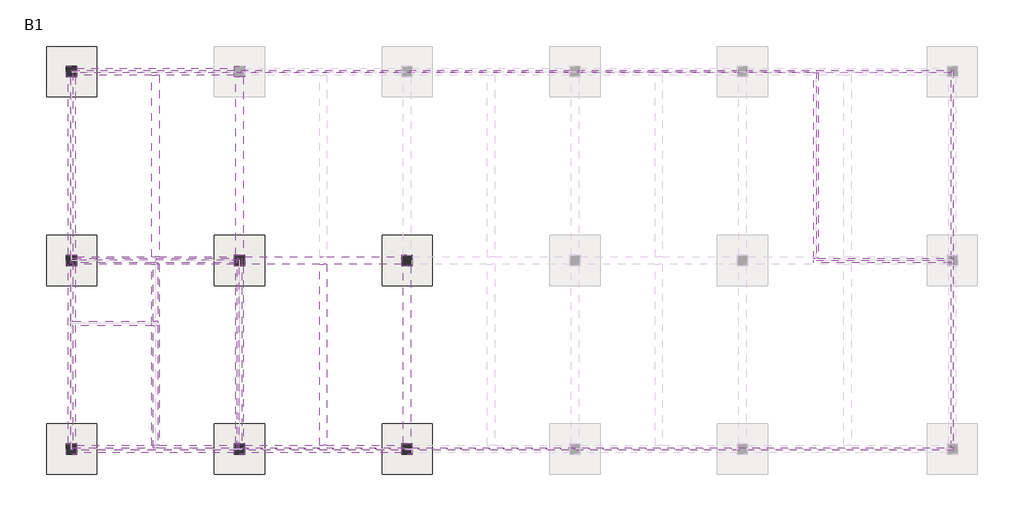
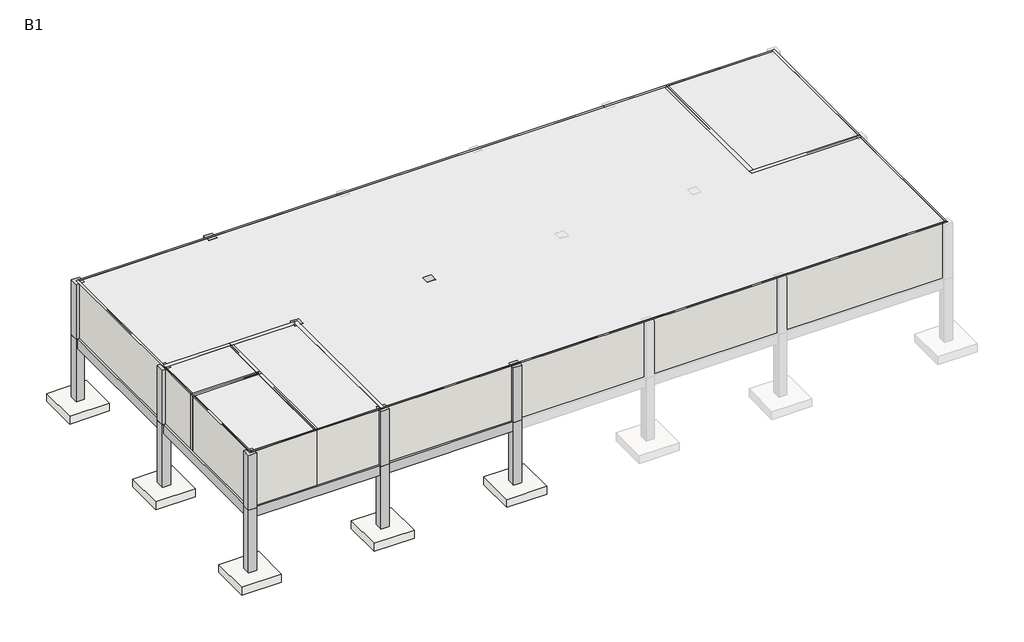
# One storey, part 1 of 2: 18 walls, 15 columns, 13 beams, 12 slabs.
"""IFC4 building model written with IfcOpenShell, lengths in millimetres."""

import ifcopenshell
import ifcopenshell.guid

model = None  # the IFC model being written
_history = None  # IfcOwnerHistory: only IFC2X3 demands one
_inside = {}  # id of a spatial element -> (the spatial element, [elements in it])
_under = {}  # id of a project, library or spatial element -> (it, [spatial elements below it])
_declared = {}  # id of a project -> (the project, [libraries it declares])
_typed = {}  # id of a type object -> (the type object, [elements of that type])
_made_of = {}  # id of a material, layer set ... -> (it, [elements and type objects made of it])


def new_model(schema):
    """Start an empty IFC model of exactly this schema.

    Asked for "IFC4X3", IfcOpenShell would pick the latest addendum, in which some entities
    have other attributes; the version numbers below select the first issue.
    IFC2X3 requires an IfcOwnerHistory on every rooted entity: one is made here for all.
    """
    global model, _history
    if schema == "IFC4X3":
        model = ifcopenshell.file(schema_version=(4, 3, 0, 0))
    else:
        model = ifcopenshell.file(schema=schema)
    _inside.clear()
    _under.clear()
    _declared.clear()
    _typed.clear()
    _made_of.clear()
    _history = None
    if model.schema == "IFC2X3":
        org = make("IfcOrganization", Name="unknown")
        user = make(
            "IfcPersonAndOrganization",
            ThePerson=make("IfcPerson", FamilyName="unknown"),
            TheOrganization=org,
        )
        app = make(
            "IfcApplication",
            ApplicationDeveloper=org,
            Version="unknown",
            ApplicationFullName="unknown",
            ApplicationIdentifier="unknown",
        )
        _history = make(
            "IfcOwnerHistory",
            OwningUser=user,
            OwningApplication=app,
            ChangeAction="ADDED",
            CreationDate=0,
        )
    return model


def make(cls, **values):
    """One entity of the class cls with the attributes given. An attribute that is None is left unset."""
    return model.create_entity(
        cls, **{name: value for name, value in values.items() if value is not None}
    )


def rooted(cls, **values):
    """An entity with a GlobalId (a new one), such as an element, a storey or a relation."""
    return make(cls, GlobalId=ifcopenshell.guid.new(), OwnerHistory=_history, **values)


def si_unit(unit_type, name, prefix=None):
    """IfcSIUnit, for example si_unit("LENGTHUNIT", "METRE", prefix="MILLI")."""
    return make("IfcSIUnit", UnitType=unit_type, Prefix=prefix, Name=name)


def assignment(units):
    """IfcUnitAssignment: the units of a project."""
    return None if units is None else make("IfcUnitAssignment", Units=units)


def point(xyz):
    """IfcCartesianPoint."""
    return None if xyz is None else make("IfcCartesianPoint", Coordinates=xyz)


def direction(xyz):
    """IfcDirection."""
    return None if xyz is None else make("IfcDirection", DirectionRatios=xyz)


def frame(location, z_axis=None, x_axis=None):
    """IfcAxis2Placement3D, a coordinate frame: its origin and axes. An axis left out is left unset."""
    return make(
        "IfcAxis2Placement3D",
        Location=point(location),
        Axis=direction(z_axis),
        RefDirection=direction(x_axis),
    )


def origin():
    """The frame at (0, 0, 0) with its axes left unset."""
    return frame((0.0, 0.0, 0.0))


def origin_with_axes():
    """The frame at (0, 0, 0) with the z axis (0, 0, 1) and the x axis (1, 0, 0) written out."""
    return frame((0.0, 0.0, 0.0), z_axis=(0.0, 0.0, 1.0), x_axis=(1.0, 0.0, 0.0))


def place(relative_to, where):
    """IfcLocalPlacement: puts the frame where relative to a parent placement (None: the world)."""
    return make(
        "IfcLocalPlacement", PlacementRelTo=relative_to, RelativePlacement=where
    )


def context(
    kind, dimensions, precision=None, world=None, true_north=None, identifier=None
):
    """IfcGeometricRepresentationContext, for example the 3D "Model" context."""
    return make(
        "IfcGeometricRepresentationContext",
        ContextIdentifier=identifier,
        ContextType=kind,
        CoordinateSpaceDimension=dimensions,
        Precision=precision,
        WorldCoordinateSystem=world,
        TrueNorth=true_north,
    )


def project(units=None, contexts=None):
    """IfcProject with its units and contexts."""
    return rooted(
        "IfcProject",
        Name="project",
        RepresentationContexts=contexts,
        UnitsInContext=assignment(units),
    )


def spatial(cls, under=None, at=None, **own):
    """A site, building, storey or space (cls), placed at a placement, below another one or the project."""
    s = rooted(cls, ObjectPlacement=at, **own)
    if under is not None:
        _under.setdefault(under.id(), (under, []))[1].append(s)
    return s


def polyline(points):
    """IfcPolyline through the points."""
    return make("IfcPolyline", Points=[point(p) for p in points])


def outline(outer, holes=None, kind="AREA"):
    """IfcArbitraryClosedProfileDef: a profile drawn as a closed curve; with holes, ...WithVoids."""
    if holes is None:
        return make("IfcArbitraryClosedProfileDef", ProfileType=kind, OuterCurve=outer)
    return make(
        "IfcArbitraryProfileDefWithVoids",
        ProfileType=kind,
        OuterCurve=outer,
        InnerCurves=holes,
    )


def extrude(swept, where, along, depth):
    """IfcExtrudedAreaSolid: the profile swept, set in the frame where, extruded along a direction by depth."""
    return make(
        "IfcExtrudedAreaSolid",
        SweptArea=swept,
        Position=where,
        ExtrudedDirection=direction(along),
        Depth=depth,
    )


def faces_of(points, faces, orient=None, outer=None):
    """IfcFace entities. A face is a list of loops; a loop is a list of indices into points, from 0.

    orient and outer hold one flag for each loop. By default every Orientation is true, the
    first loop of a face is its IfcFaceOuterBound and the others are IfcFaceBound.
    """
    made = []
    for i, loops in enumerate(faces):
        bounds = []
        for j, loop in enumerate(loops):
            is_outer = j == 0 if outer is None else outer[i][j]
            bounds.append(
                make(
                    "IfcFaceOuterBound" if is_outer else "IfcFaceBound",
                    Bound=make("IfcPolyLoop", Polygon=[points[k] for k in loop]),
                    Orientation=True if orient is None else orient[i][j],
                )
            )
        made.append(make("IfcFace", Bounds=bounds))
    return made


def faceted_brep(points, faces, orient=None, outer=None, voids=None):
    """IfcFacetedBrep: a solid bounded by flat faces; with voids (closed shells), ...WithVoids."""
    shared = [point(p) for p in points]
    hull = make("IfcClosedShell", CfsFaces=faces_of(shared, faces, orient, outer))
    if voids is None:
        return make("IfcFacetedBrep", Outer=hull)
    return make(
        "IfcFacetedBrepWithVoids",
        Outer=hull,
        Voids=[
            make(cls, CfsFaces=faces_of(shared, fs, o, b)) for cls, fs, o, b in voids
        ],
    )


def shape(context_of_items, identifier, shape_type, items):
    """IfcShapeRepresentation: the items that make up one representation, for example the "Body"."""
    return make(
        "IfcShapeRepresentation",
        ContextOfItems=context_of_items,
        RepresentationIdentifier=identifier,
        RepresentationType=shape_type,
        Items=items,
    )


def source(mapping_origin, context_of_items, identifier, shape_type, items):
    """IfcRepresentationMap: a shape defined once, which mapped items show again and again."""
    return make(
        "IfcRepresentationMap",
        MappingOrigin=mapping_origin,
        MappedRepresentation=shape(context_of_items, identifier, shape_type, items),
    )


def transform(
    local_origin,
    x_axis=None,
    y_axis=None,
    z_axis=None,
    scale=None,
    scale2=None,
    scale3=None,
    uniform=True,
):
    """IfcCartesianTransformationOperator3D, or its non-uniform kind. x_axis, y_axis, z_axis: its Axis1, 2, 3."""
    if uniform:
        return make(
            "IfcCartesianTransformationOperator3D",
            Axis1=direction(x_axis),
            Axis2=direction(y_axis),
            LocalOrigin=point(local_origin),
            Scale=scale,
            Axis3=direction(z_axis),
        )
    return make(
        "IfcCartesianTransformationOperator3DnonUniform",
        Axis1=direction(x_axis),
        Axis2=direction(y_axis),
        LocalOrigin=point(local_origin),
        Scale=scale,
        Axis3=direction(z_axis),
        Scale2=scale2,
        Scale3=scale3,
    )


def mapped(mapping_source, mapping_target):
    """IfcMappedItem: shows the shape of a source again, moved by a transform."""
    return make(
        "IfcMappedItem", MappingSource=mapping_source, MappingTarget=mapping_target
    )


def made_of(thing, what):
    """Note that an element or type object is made of a material, layer set ...; save() writes the relation."""
    if what is not None:
        _made_of.setdefault(what.id(), (what, []))[1].append(thing)
    return thing


def element(
    cls,
    number,
    at=None,
    inside=None,
    cuts=None,
    type_object=None,
    material=None,
    context=None,
    identifier="Body",
    shape_type=None,
    held_by="IfcProductDefinitionShape",
    body=None,
    shapes=None,
    **own,
):
    """One element of the class cls, such as IfcWall. Its Tag is "e" and its number.

    at: its placement. inside: the storey or other place that contains it. cuts: it is an
    opening in that element (IfcRelVoidsElement). A single representation is given by context,
    identifier, shape_type and body (its items); several are given by shapes. held_by: the class
    of the entity that holds the representations. save() writes the other relations.
    """
    e = rooted(cls, Tag="e%d" % number, ObjectPlacement=at, **own)
    if body is not None:
        shapes = [shape(context, identifier, shape_type, body)]
    if shapes is not None:
        e.Representation = make(held_by, Representations=shapes)
    if inside is not None:
        _inside.setdefault(inside.id(), (inside, []))[1].append(e)
    if cuts is not None:
        rooted(
            "IfcRelVoidsElement", RelatingBuildingElement=cuts, RelatedOpeningElement=e
        )
    if type_object is not None:
        _typed.setdefault(type_object.id(), (type_object, []))[1].append(e)
    return made_of(e, material)


def aggregate(whole, parts):
    """IfcRelAggregates: a whole, such as a stair, and the parts it consists of."""
    return rooted("IfcRelAggregates", RelatingObject=whole, RelatedObjects=parts)


def save(model, path):
    """Write the relations noted so far, then the file.

    IfcRelAggregates (storeys below a building ...), IfcRelContainedInSpatialStructure (elements
    in a storey), IfcRelDefinesByType, IfcRelAssociatesMaterial and IfcRelDeclares: one each for
    every whole, place, type object, material and project.
    """
    for whole, parts in _under.values():
        aggregate(whole, parts)
    for where, things in _inside.values():
        rooted(
            "IfcRelContainedInSpatialStructure",
            RelatedElements=things,
            RelatingStructure=where,
        )
    for kind, things in _typed.values():
        rooted("IfcRelDefinesByType", RelatedObjects=things, RelatingType=kind)
    for what, things in _made_of.values():
        rooted("IfcRelAssociatesMaterial", RelatedObjects=things, RelatingMaterial=what)
    for by, libraries in _declared.values():
        rooted("IfcRelDeclares", RelatingContext=by, RelatedDefinitions=libraries)
    model.write(path)


def ft112_footing_rectangular_ft112_2400x2400x500_5fe39465(model_context):
    return source(origin(), model_context, "Body", "SweptSolid", [
        extrude(outline(polyline([(1200.0, 1200.0), (1200.0, -1200.0), (-1200.0, -1200.0), (-1200.0, 1200.0), (1200.0, 1200.0)])), frame((0.0, 0.0, -500.0), z_axis=(0.0, 0.0, 1.0), x_axis=(1.0, 0.0, 0.0)), (0.0, 0.0, 1.0), 500.0),
    ])


model = new_model("IFC4")

# Units and contexts
model_context = context("Model", 3, world=origin())
ifc_project = project(units=[si_unit("LENGTHUNIT", "METRE", prefix="MILLI")], contexts=[model_context])

# Site, building, storey
site = spatial("IfcSite", under=ifc_project)
building = spatial("IfcBuilding", under=site)
storey = spatial("IfcBuildingStorey", under=building, Name="B1", Elevation=-4000.0)

# Beams
placement = place(None, origin())
element("IfcBeam", 1, ObjectType="Concrete-Rectangular-Beam : BM111_400x500_RG1", at=placement, inside=storey, context=model_context, shape_type="SweptSolid", body=[
    extrude(outline(polyline([(49284.6521483, 181748.8614395), (49634.6521483, 181748.8614395), (49634.6521483, 173098.8614395), (49284.6521483, 173098.8614395), (49284.6521483, 181748.8614395)])), frame((0.0, 0.0, -600.0), z_axis=(0.0, 0.0, 1.0), x_axis=(1.0, 0.0, 0.0)), (0.0, 0.0, 1.0), 600.0),
])
element("IfcBeam", 2, ObjectType="Concrete-Rectangular-Beam : BM111_400x500_RG1", at=placement, inside=storey, context=model_context, shape_type="SweptSolid", body=[
    extrude(outline(polyline([(49284.6521483, 172748.8614395), (49634.6521483, 172748.8614395), (49634.6521483, 164098.8614395), (49284.6521483, 164098.8614395), (49284.6521483, 172748.8614395)])), frame((0.0, 0.0, -600.0), z_axis=(0.0, 0.0, 1.0), x_axis=(1.0, 0.0, 0.0)), (0.0, 0.0, 1.0), 600.0),
])
element("IfcBeam", 3, ObjectType="Concrete-Rectangular-Beam : BM111_400x500_RG1", at=placement, inside=storey, context=model_context, shape_type="SweptSolid", body=[
    extrude(outline(polyline([(57284.6521483, 172748.8614395), (57634.6521483, 172748.8614395), (57634.6521483, 164098.8614395), (57284.6521483, 164098.8614395), (57284.6521483, 172748.8614395)])), frame((0.0, 0.0, -600.0), z_axis=(0.0, 0.0, 1.0), x_axis=(1.0, 0.0, 0.0)), (0.0, 0.0, 1.0), 600.0),
])
element("IfcBeam", 4, ObjectType="Concrete-Rectangular-Beam : BM111_400x500_RG1", at=placement, inside=storey, context=model_context, shape_type="Brep", body=[
    faceted_brep([(45709.6521483, 182098.8614395, 0.0), (45709.6521483, 181748.8614395, 0.0), (49284.6521483, 181748.8614395, 0.0), (49634.6521483, 181748.8614395, 0.0), (53209.6521483, 181748.8614395, 0.0), (53209.6521483, 182098.8614395, 0.0), (45709.6521483, 181748.8614395, -600.0), (49284.6521483, 181748.8614395, -600.0), (49634.6521483, 181748.8614395, -600.0), (53209.6521483, 181748.8614395, -600.0), (45709.6521483, 182098.8614395, -600.0), (53209.6521483, 182098.8614395, -600.0)], [[[0, 1, 2, 3, 4, 5]], [[1, 6, 7, 8, 9, 4, 3, 2]], [[6, 10, 11, 9, 8, 7]], [[10, 0, 5, 11]], [[1, 0, 10, 6]], [[5, 4, 9, 11]]]),
])
element("IfcBeam", 5, ObjectType="Concrete-Rectangular-Beam : BM111_400x500_RG1", at=placement, inside=storey, context=model_context, shape_type="Brep", body=[
    faceted_brep([(45709.6521483, 173098.8614395, 0.0), (45709.6521483, 172748.8614395, 0.0), (49284.6521483, 172748.8614395, 0.0), (49634.6521483, 172748.8614395, 0.0), (53209.6521483, 172748.8614395, 0.0), (53209.6521483, 173098.8614395, 0.0), (49634.6521483, 173098.8614395, 0.0), (49284.6521483, 173098.8614395, 0.0), (45709.6521483, 172748.8614395, -600.0), (49284.6521483, 172748.8614395, -600.0), (49634.6521483, 172748.8614395, -600.0), (53209.6521483, 172748.8614395, -600.0), (45709.6521483, 173098.8614395, -600.0), (49284.6521483, 173098.8614395, -600.0), (49634.6521483, 173098.8614395, -600.0), (53209.6521483, 173098.8614395, -600.0)], [[[0, 1, 2, 3, 4, 5, 6, 7]], [[1, 8, 9, 10, 11, 4, 3, 2]], [[8, 12, 13, 14, 15, 11, 10, 9]], [[12, 0, 7, 6, 5, 15, 14, 13]], [[1, 0, 12, 8]], [[5, 4, 11, 15]]]),
])
element("IfcBeam", 6, ObjectType="Concrete-Rectangular-Beam : BM111_400x500_RG1", at=placement, inside=storey, context=model_context, shape_type="Brep", body=[
    faceted_brep([(53709.6521483, 173098.8614395, 0.0), (53709.6521483, 172748.8614395, 0.0), (57284.6521483, 172748.8614395, 0.0), (57634.6521483, 172748.8614395, 0.0), (61209.6521483, 172748.8614395, 0.0), (61209.6521483, 173098.8614395, 0.0), (57634.6521483, 173098.8614395, 0.0), (57284.6521483, 173098.8614395, 0.0), (53709.6521483, 172748.8614395, -600.0), (57284.6521483, 172748.8614395, -600.0), (57634.6521483, 172748.8614395, -600.0), (61209.6521483, 172748.8614395, -600.0), (53709.6521483, 173098.8614395, -600.0), (57284.6521483, 173098.8614395, -600.0), (57634.6521483, 173098.8614395, -600.0), (61209.6521483, 173098.8614395, -600.0)], [[[0, 1, 2, 3, 4, 5, 6, 7]], [[1, 8, 9, 10, 11, 4, 3, 2]], [[8, 12, 13, 14, 15, 11, 10, 9]], [[12, 0, 7, 6, 5, 15, 14, 13]], [[1, 0, 12, 8]], [[5, 4, 11, 15]]]),
])
element("IfcBeam", 7, ObjectType="Concrete-Rectangular-Beam : BM111_400x500_RG1", at=placement, inside=storey, context=model_context, shape_type="Brep", body=[
    faceted_brep([(45709.6521483, 164098.8614395, 0.0), (45709.6521483, 163748.8614395, 0.0), (53209.6521483, 163748.8614395, 0.0), (53209.6521483, 164098.8614395, 0.0), (49634.6521483, 164098.8614395, 0.0), (49284.6521483, 164098.8614395, 0.0), (45709.6521483, 163748.8614395, -600.0), (53209.6521483, 163748.8614395, -600.0), (45709.6521483, 164098.8614395, -600.0), (49284.6521483, 164098.8614395, -600.0), (49634.6521483, 164098.8614395, -600.0), (53209.6521483, 164098.8614395, -600.0)], [[[0, 1, 2, 3, 4, 5]], [[1, 6, 7, 2]], [[6, 8, 9, 10, 11, 7]], [[8, 0, 5, 4, 3, 11, 10, 9]], [[1, 0, 8, 6]], [[3, 2, 7, 11]]]),
])
element("IfcBeam", 8, ObjectType="Concrete-Rectangular-Beam : BM111_400x500_RG1", at=placement, inside=storey, context=model_context, shape_type="Brep", body=[
    faceted_brep([(53709.6521483, 164098.8614395, 0.0), (53709.6521483, 163748.8614395, 0.0), (61209.6521483, 163748.8614395, 0.0), (61209.6521483, 164098.8614395, 0.0), (57634.6521483, 164098.8614395, 0.0), (57284.6521483, 164098.8614395, 0.0), (53709.6521483, 163748.8614395, -600.0), (61209.6521483, 163748.8614395, -600.0), (53709.6521483, 164098.8614395, -600.0), (57284.6521483, 164098.8614395, -600.0), (57634.6521483, 164098.8614395, -600.0), (61209.6521483, 164098.8614395, -600.0)], [[[0, 1, 2, 3, 4, 5]], [[1, 6, 7, 2]], [[6, 8, 9, 10, 11, 7]], [[8, 0, 5, 4, 3, 11, 10, 9]], [[1, 0, 8, 6]], [[3, 2, 7, 11]]]),
])
element("IfcBeam", 9, ObjectType="Concrete-Rectangular-Beam : BM111_400x500_RG1", at=placement, inside=storey, context=model_context, shape_type="SweptSolid", body=[
    extrude(outline(polyline([(45284.6521483, 181673.8614395), (45634.6521483, 181673.8614395), (45634.6521483, 173173.8614395), (45284.6521483, 173173.8614395), (45284.6521483, 181673.8614395)])), frame((0.0, 0.0, -600.0), z_axis=(0.0, 0.0, 1.0), x_axis=(1.0, 0.0, 0.0)), (0.0, 0.0, 1.0), 600.0),
])
element("IfcBeam", 10, ObjectType="Concrete-Rectangular-Beam : BM111_400x500_RG1", at=placement, inside=storey, context=model_context, shape_type="SweptSolid", body=[
    extrude(outline(polyline([(45284.6521483, 172673.8614395), (45634.6521483, 172673.8614395), (45634.6521483, 164173.8614395), (45284.6521483, 164173.8614395), (45284.6521483, 172673.8614395)])), frame((0.0, 0.0, -600.0), z_axis=(0.0, 0.0, 1.0), x_axis=(1.0, 0.0, 0.0)), (0.0, 0.0, 1.0), 600.0),
])
element("IfcBeam", 11, ObjectType="Concrete-Rectangular-Beam : BM111_400x500_RG1", at=placement, inside=storey, context=model_context, shape_type="SweptSolid", body=[
    extrude(outline(polyline([(53284.6521483, 181673.8614395), (53634.6521483, 181673.8614395), (53634.6521483, 173173.8614395), (53284.6521483, 173173.8614395), (53284.6521483, 181673.8614395)])), frame((0.0, 0.0, -600.0), z_axis=(0.0, 0.0, 1.0), x_axis=(1.0, 0.0, 0.0)), (0.0, 0.0, 1.0), 600.0),
])
element("IfcBeam", 12, ObjectType="Concrete-Rectangular-Beam : BM111_400x500_RG1", at=placement, inside=storey, context=model_context, shape_type="SweptSolid", body=[
    extrude(outline(polyline([(53284.6521483, 172673.8614395), (53634.6521483, 172673.8614395), (53634.6521483, 164173.8614395), (53284.6521483, 164173.8614395), (53284.6521483, 172673.8614395)])), frame((0.0, 0.0, -600.0), z_axis=(0.0, 0.0, 1.0), x_axis=(1.0, 0.0, 0.0)), (0.0, 0.0, 1.0), 600.0),
])
element("IfcBeam", 13, ObjectType="Concrete-Rectangular-Beam : BM111_400x500_RG1", at=placement, inside=storey, context=model_context, shape_type="SweptSolid", body=[
    extrude(outline(polyline([(61284.6521483, 172673.8614395), (61634.6521483, 172673.8614395), (61634.6521483, 164173.8614395), (61284.6521483, 164173.8614395), (61284.6521483, 172673.8614395)])), frame((0.0, 0.0, -600.0), z_axis=(0.0, 0.0, 1.0), x_axis=(1.0, 0.0, 0.0)), (0.0, 0.0, 1.0), 600.0),
])

# Columns
element("IfcColumn", 14, ObjectType="Concrete-Rectangular-Column : CL111_500x500", at=placement, inside=storey, context=model_context, shape_type="Brep", body=[
    faceted_brep([(45709.6521483, 182173.8614395, 0.0), (45709.6521483, 181673.8614395, 0.0), (45209.6521483, 181673.8614395, 0.0), (45209.6521483, 182173.8614395, 0.0), (45709.6521483, 182173.8614395, 3500.0), (45709.6521483, 182098.8614395, 3500.0), (45709.6521483, 181748.8614395, 3500.0), (45709.6521483, 181673.8614395, 3500.0), (45634.6521483, 181673.8614395, 3500.0), (45284.6521483, 181673.8614395, 3500.0), (45209.6521483, 181673.8614395, 3500.0), (45209.6521483, 182173.8614395, 3500.0)], [[[0, 1, 2, 3]], [[4, 5, 6, 7, 1, 0]], [[7, 8, 9, 10, 2, 1]], [[10, 11, 3, 2]], [[11, 4, 0, 3]], [[4, 11, 10, 9, 8, 7, 6, 5]]]),
])
element("IfcColumn", 15, ObjectType="Concrete-Rectangular-Column : CL111_500x500", at=placement, inside=storey, context=model_context, shape_type="Brep", body=[
    faceted_brep([(53709.6521483, 182173.8614395, 0.0), (53709.6521483, 181673.8614395, 0.0), (53209.6521483, 181673.8614395, 0.0), (53209.6521483, 182173.8614395, 0.0), (53709.6521483, 182173.8614395, 3500.0), (53709.6521483, 182098.8614395, 3500.0), (53709.6521483, 181748.8614395, 3500.0), (53709.6521483, 181673.8614395, 3500.0), (53634.6521483, 181673.8614395, 3500.0), (53284.6521483, 181673.8614395, 3500.0), (53209.6521483, 181673.8614395, 3500.0), (53209.6521483, 181748.8614395, 3500.0), (53209.6521483, 182098.8614395, 3500.0), (53209.6521483, 182173.8614395, 3500.0)], [[[0, 1, 2, 3]], [[4, 5, 6, 7, 1, 0]], [[7, 8, 9, 10, 2, 1]], [[10, 11, 12, 13, 3, 2]], [[13, 4, 0, 3]], [[4, 13, 12, 11, 10, 9, 8, 7, 6, 5]]]),
])
element("IfcColumn", 16, ObjectType="Concrete-Rectangular-Column : CL111_500x500", at=placement, inside=storey, context=model_context, shape_type="Brep", body=[
    faceted_brep([(45709.6521483, 173173.8614395, 0.0), (45709.6521483, 172673.8614395, 0.0), (45209.6521483, 172673.8614395, 0.0), (45209.6521483, 173173.8614395, 0.0), (45709.6521483, 173173.8614395, 3500.0), (45709.6521483, 173098.8614395, 3500.0), (45709.6521483, 172748.8614395, 3500.0), (45709.6521483, 172673.8614395, 3500.0), (45634.6521483, 172673.8614395, 3500.0), (45284.6521483, 172673.8614395, 3500.0), (45209.6521483, 172673.8614395, 3500.0), (45209.6521483, 173173.8614395, 3500.0), (45284.6521483, 173173.8614395, 3500.0), (45634.6521483, 173173.8614395, 3500.0)], [[[0, 1, 2, 3]], [[4, 5, 6, 7, 1, 0]], [[7, 8, 9, 10, 2, 1]], [[10, 11, 3, 2]], [[11, 12, 13, 4, 0, 3]], [[4, 13, 12, 11, 10, 9, 8, 7, 6, 5]]]),
])
element("IfcColumn", 17, ObjectType="Concrete-Rectangular-Column : CL111_500x500", at=placement, inside=storey, context=model_context, shape_type="Brep", body=[
    faceted_brep([(53709.6521483, 173173.8614395, 0.0), (53709.6521483, 172673.8614395, 0.0), (53209.6521483, 172673.8614395, 0.0), (53209.6521483, 173173.8614395, 0.0), (53709.6521483, 173173.8614395, 3500.0), (53709.6521483, 173098.8614395, 3500.0), (53709.6521483, 172748.8614395, 3500.0), (53709.6521483, 172673.8614395, 3500.0), (53634.6521483, 172673.8614395, 3500.0), (53284.6521483, 172673.8614395, 3500.0), (53209.6521483, 172673.8614395, 3500.0), (53209.6521483, 172748.8614395, 3500.0), (53209.6521483, 173098.8614395, 3500.0), (53209.6521483, 173173.8614395, 3500.0), (53284.6521483, 173173.8614395, 3500.0), (53634.6521483, 173173.8614395, 3500.0)], [[[0, 1, 2, 3]], [[4, 5, 6, 7, 1, 0]], [[7, 8, 9, 10, 2, 1]], [[10, 11, 12, 13, 3, 2]], [[13, 14, 15, 4, 0, 3]], [[4, 15, 14, 13, 12, 11, 10, 9, 8, 7, 6, 5]]]),
])
element("IfcColumn", 18, ObjectType="Concrete-Rectangular-Column : CL111_500x500", at=placement, inside=storey, context=model_context, shape_type="Brep", body=[
    faceted_brep([(61709.6521483, 173173.8614395, 0.0), (61709.6521483, 172673.8614395, 0.0), (61209.6521483, 172673.8614395, 0.0), (61209.6521483, 173173.8614395, 0.0), (61709.6521483, 173173.8614395, 3500.0), (61709.6521483, 173098.8614395, 3500.0), (61709.6521483, 172748.8614395, 3500.0), (61709.6521483, 172673.8614395, 3500.0), (61634.6521483, 172673.8614395, 3500.0), (61284.6521483, 172673.8614395, 3500.0), (61209.6521483, 172673.8614395, 3500.0), (61209.6521483, 172748.8614395, 3500.0), (61209.6521483, 173098.8614395, 3500.0), (61209.6521483, 173173.8614395, 3500.0), (61284.6521483, 173173.8614395, 3500.0), (61634.6521483, 173173.8614395, 3500.0)], [[[0, 1, 2, 3]], [[4, 5, 6, 7, 1, 0]], [[7, 8, 9, 10, 2, 1]], [[10, 11, 12, 13, 3, 2]], [[13, 14, 15, 4, 0, 3]], [[4, 15, 14, 13, 12, 11, 10, 9, 8, 7, 6, 5]]]),
])
element("IfcColumn", 19, ObjectType="Concrete-Rectangular-Column : CL111_500x500", at=placement, inside=storey, context=model_context, shape_type="Brep", body=[
    faceted_brep([(45709.6521483, 164173.8614395, 0.0), (45709.6521483, 163673.8614395, 0.0), (45209.6521483, 163673.8614395, 0.0), (45209.6521483, 164173.8614395, 0.0), (45709.6521483, 164173.8614395, 3500.0), (45709.6521483, 164098.8614395, 3500.0), (45709.6521483, 163748.8614395, 3500.0), (45709.6521483, 163673.8614395, 3500.0), (45209.6521483, 163673.8614395, 3500.0), (45209.6521483, 164173.8614395, 3500.0), (45284.6521483, 164173.8614395, 3500.0), (45634.6521483, 164173.8614395, 3500.0)], [[[0, 1, 2, 3]], [[4, 5, 6, 7, 1, 0]], [[7, 8, 2, 1]], [[8, 9, 3, 2]], [[9, 10, 11, 4, 0, 3]], [[4, 11, 10, 9, 8, 7, 6, 5]]]),
])
element("IfcColumn", 20, ObjectType="Concrete-Rectangular-Column : CL111_500x500", at=placement, inside=storey, context=model_context, shape_type="Brep", body=[
    faceted_brep([(53709.6521483, 164173.8614395, 0.0), (53709.6521483, 163673.8614395, 0.0), (53209.6521483, 163673.8614395, 0.0), (53209.6521483, 164173.8614395, 0.0), (53709.6521483, 164173.8614395, 3500.0), (53709.6521483, 164098.8614395, 3500.0), (53709.6521483, 163748.8614395, 3500.0), (53709.6521483, 163673.8614395, 3500.0), (53209.6521483, 163673.8614395, 3500.0), (53209.6521483, 163748.8614395, 3500.0), (53209.6521483, 164098.8614395, 3500.0), (53209.6521483, 164173.8614395, 3500.0), (53284.6521483, 164173.8614395, 3500.0), (53634.6521483, 164173.8614395, 3500.0)], [[[0, 1, 2, 3]], [[4, 5, 6, 7, 1, 0]], [[7, 8, 2, 1]], [[8, 9, 10, 11, 3, 2]], [[11, 12, 13, 4, 0, 3]], [[4, 13, 12, 11, 10, 9, 8, 7, 6, 5]]]),
])
element("IfcColumn", 21, ObjectType="Concrete-Rectangular-Column : CL111_500x500", at=placement, inside=storey, context=model_context, shape_type="Brep", body=[
    faceted_brep([(61709.6521483, 164173.8614395, 0.0), (61709.6521483, 163673.8614395, 0.0), (61209.6521483, 163673.8614395, 0.0), (61209.6521483, 164173.8614395, 0.0), (61709.6521483, 164173.8614395, 3500.0), (61709.6521483, 164098.8614395, 3500.0), (61709.6521483, 163748.8614395, 3500.0), (61709.6521483, 163673.8614395, 3500.0), (61209.6521483, 163673.8614395, 3500.0), (61209.6521483, 163748.8614395, 3500.0), (61209.6521483, 164098.8614395, 3500.0), (61209.6521483, 164173.8614395, 3500.0), (61284.6521483, 164173.8614395, 3500.0), (61634.6521483, 164173.8614395, 3500.0)], [[[0, 1, 2, 3]], [[4, 5, 6, 7, 1, 0]], [[7, 8, 2, 1]], [[8, 9, 10, 11, 3, 2]], [[11, 12, 13, 4, 0, 3]], [[4, 13, 12, 11, 10, 9, 8, 7, 6, 5]]]),
])
element("IfcColumn", 22, ObjectType="Concrete-Rectangular-Column : CL111_500x500", at=placement, inside=storey, context=model_context, shape_type="Brep", body=[
    faceted_brep([(45709.6521483, 182173.8614395, -4000.0), (45709.6521483, 181673.8614395, -4000.0), (45209.6521483, 181673.8614395, -4000.0), (45209.6521483, 182173.8614395, -4000.0), (45709.6521483, 182173.8614395, 0.0), (45709.6521483, 182098.8614395, 0.0), (45709.6521483, 181748.8614395, 0.0), (45709.6521483, 181673.8614395, 0.0), (45634.6521483, 181673.8614395, 0.0), (45284.6521483, 181673.8614395, 0.0), (45209.6521483, 181673.8614395, 0.0), (45209.6521483, 182173.8614395, 0.0)], [[[0, 1, 2, 3]], [[4, 5, 6, 7, 1, 0]], [[7, 8, 9, 10, 2, 1]], [[10, 11, 3, 2]], [[11, 4, 0, 3]], [[4, 11, 10, 9, 8, 7, 6, 5]]]),
])
element("IfcColumn", 23, ObjectType="Concrete-Rectangular-Column : CL111_500x500", at=placement, inside=storey, context=model_context, shape_type="Brep", body=[
    faceted_brep([(45709.6521483, 173173.8614395, -4000.0), (45709.6521483, 172673.8614395, -4000.0), (45209.6521483, 172673.8614395, -4000.0), (45209.6521483, 173173.8614395, -4000.0), (45709.6521483, 173173.8614395, 0.0), (45709.6521483, 173098.8614395, 0.0), (45709.6521483, 172748.8614395, 0.0), (45709.6521483, 172673.8614395, 0.0), (45634.6521483, 172673.8614395, 0.0), (45284.6521483, 172673.8614395, 0.0), (45209.6521483, 172673.8614395, 0.0), (45209.6521483, 173173.8614395, 0.0), (45284.6521483, 173173.8614395, 0.0), (45634.6521483, 173173.8614395, 0.0)], [[[0, 1, 2, 3]], [[4, 5, 6, 7, 1, 0]], [[7, 8, 9, 10, 2, 1]], [[10, 11, 3, 2]], [[11, 12, 13, 4, 0, 3]], [[4, 13, 12, 11, 10, 9, 8, 7, 6, 5]]]),
])
element("IfcColumn", 24, ObjectType="Concrete-Rectangular-Column : CL111_500x500", at=placement, inside=storey, context=model_context, shape_type="Brep", body=[
    faceted_brep([(53709.6521483, 173173.8614395, -4000.0), (53709.6521483, 172673.8614395, -4000.0), (53209.6521483, 172673.8614395, -4000.0), (53209.6521483, 173173.8614395, -4000.0), (53709.6521483, 173173.8614395, 0.0), (53709.6521483, 173098.8614395, 0.0), (53709.6521483, 172748.8614395, 0.0), (53709.6521483, 172673.8614395, 0.0), (53634.6521483, 172673.8614395, 0.0), (53284.6521483, 172673.8614395, 0.0), (53209.6521483, 172673.8614395, 0.0), (53209.6521483, 172748.8614395, 0.0), (53209.6521483, 173098.8614395, 0.0), (53209.6521483, 173173.8614395, 0.0), (53284.6521483, 173173.8614395, 0.0), (53634.6521483, 173173.8614395, 0.0)], [[[0, 1, 2, 3]], [[4, 5, 6, 7, 1, 0]], [[7, 8, 9, 10, 2, 1]], [[10, 11, 12, 13, 3, 2]], [[13, 14, 15, 4, 0, 3]], [[4, 15, 14, 13, 12, 11, 10, 9, 8, 7, 6, 5]]]),
])
element("IfcColumn", 25, ObjectType="Concrete-Rectangular-Column : CL111_500x500", at=placement, inside=storey, context=model_context, shape_type="Brep", body=[
    faceted_brep([(61709.6521483, 173173.8614395, -4000.0), (61709.6521483, 172673.8614395, -4000.0), (61209.6521483, 172673.8614395, -4000.0), (61209.6521483, 173173.8614395, -4000.0), (61709.6521483, 173173.8614395, 0.0), (61709.6521483, 173098.8614395, 0.0), (61709.6521483, 172748.8614395, 0.0), (61709.6521483, 172673.8614395, 0.0), (61634.6521483, 172673.8614395, 0.0), (61284.6521483, 172673.8614395, 0.0), (61209.6521483, 172673.8614395, 0.0), (61209.6521483, 172748.8614395, 0.0), (61209.6521483, 173098.8614395, 0.0), (61209.6521483, 173173.8614395, 0.0), (61284.6521483, 173173.8614395, 0.0), (61634.6521483, 173173.8614395, 0.0)], [[[0, 1, 2, 3]], [[4, 5, 6, 7, 1, 0]], [[7, 8, 9, 10, 2, 1]], [[10, 11, 12, 13, 3, 2]], [[13, 14, 15, 4, 0, 3]], [[4, 15, 14, 13, 12, 11, 10, 9, 8, 7, 6, 5]]]),
])
element("IfcColumn", 26, ObjectType="Concrete-Rectangular-Column : CL111_500x500", at=placement, inside=storey, context=model_context, shape_type="Brep", body=[
    faceted_brep([(45709.6521483, 164173.8614395, -4000.0), (45709.6521483, 163673.8614395, -4000.0), (45209.6521483, 163673.8614395, -4000.0), (45209.6521483, 164173.8614395, -4000.0), (45709.6521483, 164173.8614395, 0.0), (45709.6521483, 164098.8614395, 0.0), (45709.6521483, 163748.8614395, 0.0), (45709.6521483, 163673.8614395, 0.0), (45209.6521483, 163673.8614395, 0.0), (45209.6521483, 164173.8614395, 0.0), (45284.6521483, 164173.8614395, 0.0), (45634.6521483, 164173.8614395, 0.0)], [[[0, 1, 2, 3]], [[4, 5, 6, 7, 1, 0]], [[7, 8, 2, 1]], [[8, 9, 3, 2]], [[9, 10, 11, 4, 0, 3]], [[4, 11, 10, 9, 8, 7, 6, 5]]]),
])
element("IfcColumn", 27, ObjectType="Concrete-Rectangular-Column : CL111_500x500", at=placement, inside=storey, context=model_context, shape_type="Brep", body=[
    faceted_brep([(53709.6521483, 164173.8614395, -4000.0), (53709.6521483, 163673.8614395, -4000.0), (53209.6521483, 163673.8614395, -4000.0), (53209.6521483, 164173.8614395, -4000.0), (53709.6521483, 164173.8614395, 0.0), (53709.6521483, 164098.8614395, 0.0), (53709.6521483, 163748.8614395, 0.0), (53709.6521483, 163673.8614395, 0.0), (53209.6521483, 163673.8614395, 0.0), (53209.6521483, 163748.8614395, 0.0), (53209.6521483, 164098.8614395, 0.0), (53209.6521483, 164173.8614395, 0.0), (53284.6521483, 164173.8614395, 0.0), (53634.6521483, 164173.8614395, 0.0)], [[[0, 1, 2, 3]], [[4, 5, 6, 7, 1, 0]], [[7, 8, 2, 1]], [[8, 9, 10, 11, 3, 2]], [[11, 12, 13, 4, 0, 3]], [[4, 13, 12, 11, 10, 9, 8, 7, 6, 5]]]),
])
element("IfcColumn", 28, ObjectType="Concrete-Rectangular-Column : CL111_500x500", at=placement, inside=storey, context=model_context, shape_type="Brep", body=[
    faceted_brep([(61709.6521483, 164173.8614395, -4000.0), (61709.6521483, 163673.8614395, -4000.0), (61209.6521483, 163673.8614395, -4000.0), (61209.6521483, 164173.8614395, -4000.0), (61709.6521483, 164173.8614395, 0.0), (61709.6521483, 164098.8614395, 0.0), (61709.6521483, 163748.8614395, 0.0), (61709.6521483, 163673.8614395, 0.0), (61209.6521483, 163673.8614395, 0.0), (61209.6521483, 163748.8614395, 0.0), (61209.6521483, 164098.8614395, 0.0), (61209.6521483, 164173.8614395, 0.0), (61284.6521483, 164173.8614395, 0.0), (61634.6521483, 164173.8614395, 0.0)], [[[0, 1, 2, 3]], [[4, 5, 6, 7, 1, 0]], [[7, 8, 2, 1]], [[8, 9, 10, 11, 3, 2]], [[11, 12, 13, 4, 0, 3]], [[4, 13, 12, 11, 10, 9, 8, 7, 6, 5]]]),
])

# Slabs
element("IfcSlab", 29, ObjectType="CFS11_Slab RC_T150", at=placement, inside=storey, context=model_context, shape_type="SweptSolid", body=[
    extrude(outline(polyline([(87459.6521483, 181923.8614395), (87459.6521483, 172923.8614395), (80959.6521483, 172923.8614395), (80959.6521483, 181923.8614395), (87459.6521483, 181923.8614395)])), frame((0.0, 0.0, -150.0), z_axis=(0.0, 0.0, 1.0), x_axis=(1.0, 0.0, 0.0)), (0.0, 0.0, 1.0), 150.0),
])
element("IfcSlab", 30, ObjectType="CFS11_Slab RC_T150", at=placement, inside=storey, context=model_context, shape_type="SweptSolid", body=[
    extrude(outline(polyline([(53459.6521483, 163923.8614395), (49459.6521483, 163923.8614395), (49459.6521483, 172923.8614395), (53459.6521483, 172923.8614395), (53459.6521483, 163923.8614395)])), frame((0.0, 0.0, -150.0), z_axis=(0.0, 0.0, 1.0), x_axis=(1.0, 0.0, 0.0)), (0.0, 0.0, 1.0), 150.0),
])
element("IfcSlab", 31, ObjectType="CFS11_Slab RC_T150", at=placement, inside=storey, context=model_context, shape_type="SweptSolid", body=[
    extrude(outline(polyline([(80959.6521483, 181923.8614395), (80959.6521483, 172923.8614395), (87459.6521483, 172923.8614395), (87459.6521483, 163923.8614395), (53459.6521483, 163923.8614395), (53459.6521483, 172923.8614395), (45459.6521483, 172923.8614395), (45459.6521483, 181923.8614395), (80959.6521483, 181923.8614395)])), frame((0.0, 0.0, -150.0), z_axis=(0.0, 0.0, 1.0), x_axis=(1.0, 0.0, 0.0)), (0.0, 0.0, 1.0), 150.0),
])
element("IfcSlab", 32, ObjectType="CFS11_Slab RC_T150", at=placement, inside=storey, context=model_context, shape_type="SweptSolid", body=[
    extrude(outline(polyline([(45459.6521483, 163923.8614395), (45459.6521483, 169923.8614395), (49459.6521483, 169923.8614395), (49459.6521483, 163923.8614395), (45459.6521483, 163923.8614395)])), frame((0.0, 0.0, -150.0), z_axis=(0.0, 0.0, 1.0), x_axis=(1.0, 0.0, 0.0)), (0.0, 0.0, 1.0), 150.0),
])
element("IfcSlab", 33, ObjectType="CFS11_Slab RC_T150", at=placement, inside=storey, context=model_context, shape_type="SweptSolid", body=[
    extrude(outline(polyline([(45459.6521483, 172923.8614395), (49459.6521483, 172923.8614395), (49459.6521483, 169923.8614395), (45459.6521483, 169923.8614395), (45459.6521483, 172923.8614395)])), frame((0.0, 0.0, -150.0), z_axis=(0.0, 0.0, 1.0), x_axis=(1.0, 0.0, 0.0)), (0.0, 0.0, 1.0), 150.0),
])
ft112_footing_rectangular_ft112_2400x2400x500_shape = ft112_footing_rectangular_ft112_2400x2400x500_5fe39465(model_context)
element("IfcSlab", 34, ObjectType="FT112-Footing-Rectangular : FT112_2400x2400x500", at=placement, inside=storey, context=model_context, shape_type="MappedRepresentation", body=[
    mapped(ft112_footing_rectangular_ft112_2400x2400x500_shape, transform((45459.6521483, 181923.8614395, -4000.0), x_axis=(1.0, 0.0, 0.0), y_axis=(0.0, 1.0, 0.0), z_axis=(0.0, 0.0, 1.0))),
])
element("IfcSlab", 35, ObjectType="FT112-Footing-Rectangular : FT112_2400x2400x500", at=placement, inside=storey, context=model_context, shape_type="MappedRepresentation", body=[
    mapped(ft112_footing_rectangular_ft112_2400x2400x500_shape, transform((45459.6521483, 172923.8614395, -4000.0), x_axis=(1.0, 0.0, 0.0), y_axis=(0.0, 1.0, 0.0), z_axis=(0.0, 0.0, 1.0))),
])
element("IfcSlab", 36, ObjectType="FT112-Footing-Rectangular : FT112_2400x2400x500", at=placement, inside=storey, context=model_context, shape_type="MappedRepresentation", body=[
    mapped(ft112_footing_rectangular_ft112_2400x2400x500_shape, transform((53459.6521483, 172923.8614395, -4000.0), x_axis=(1.0, 0.0, 0.0), y_axis=(0.0, 1.0, 0.0), z_axis=(0.0, 0.0, 1.0))),
])
element("IfcSlab", 37, ObjectType="FT112-Footing-Rectangular : FT112_2400x2400x500", at=placement, inside=storey, context=model_context, shape_type="MappedRepresentation", body=[
    mapped(ft112_footing_rectangular_ft112_2400x2400x500_shape, transform((61459.6521483, 172923.8614395, -4000.0), x_axis=(1.0, 0.0, 0.0), y_axis=(0.0, 1.0, 0.0), z_axis=(0.0, 0.0, 1.0))),
])
element("IfcSlab", 38, ObjectType="FT112-Footing-Rectangular : FT112_2400x2400x500", at=placement, inside=storey, context=model_context, shape_type="MappedRepresentation", body=[
    mapped(ft112_footing_rectangular_ft112_2400x2400x500_shape, transform((45459.6521483, 163923.8614395, -4000.0), x_axis=(1.0, 0.0, 0.0), y_axis=(0.0, 1.0, 0.0), z_axis=(0.0, 0.0, 1.0))),
])
element("IfcSlab", 39, ObjectType="FT112-Footing-Rectangular : FT112_2400x2400x500", at=placement, inside=storey, context=model_context, shape_type="MappedRepresentation", body=[
    mapped(ft112_footing_rectangular_ft112_2400x2400x500_shape, transform((53459.6521483, 163923.8614395, -4000.0), x_axis=(1.0, 0.0, 0.0), y_axis=(0.0, 1.0, 0.0), z_axis=(0.0, 0.0, 1.0))),
])
element("IfcSlab", 40, ObjectType="FT112-Footing-Rectangular : FT112_2400x2400x500", at=placement, inside=storey, context=model_context, shape_type="MappedRepresentation", body=[
    mapped(ft112_footing_rectangular_ft112_2400x2400x500_shape, transform((61459.6521483, 163923.8614395, -4000.0), x_axis=(1.0, 0.0, 0.0), y_axis=(0.0, 1.0, 0.0), z_axis=(0.0, 0.0, 1.0))),
])

# Walls
element("IfcWall", 41, ObjectType="WA211_Exterior-Cement Brick-90mm", at=placement, inside=storey, context=model_context, shape_type="Brep", body=[
    faceted_brep([(80959.6521483, 181866.8614395, 0.0), (81066.6521483, 181866.8614395, 0.0), (87402.6521483, 181866.8614395, 0.0), (87402.6521483, 181866.8614395, 3500.0), (81066.6521483, 181866.8614395, 3500.0), (80959.6521483, 181866.8614395, 3500.0), (80959.6521483, 181980.8614395, 0.0), (80959.6521483, 181980.8614395, 3500.0), (87402.6521483, 181980.8614395, 3500.0), (87402.6521483, 181980.8614395, 0.0)], [[[0, 1, 2, 3, 4, 5]], [[6, 7, 8, 9]], [[2, 1, 0, 6, 9]], [[5, 4, 3, 8, 7]], [[0, 5, 7, 6]], [[3, 2, 9, 8]]]),
])
element("IfcWall", 42, ObjectType="WA211_Exterior-Cement Brick-90mm", at=placement, inside=storey, context=model_context, shape_type="Brep", body=[
    faceted_brep([(87402.6521483, 181980.8614395, 0.0), (87402.6521483, 181866.8614395, 0.0), (87402.6521483, 173030.8614395, 0.0), (87402.6521483, 173030.8614395, 3500.0), (87402.6521483, 181866.8614395, 3500.0), (87402.6521483, 181980.8614395, 3500.0), (87516.6521483, 181980.8614395, 0.0), (87516.6521483, 181980.8614395, 3500.0), (87516.6521483, 173030.8614395, 3500.0), (87516.6521483, 173030.8614395, 0.0)], [[[0, 1, 2, 3, 4, 5]], [[6, 7, 8, 9]], [[2, 1, 0, 6, 9]], [[5, 4, 3, 8, 7]], [[0, 5, 7, 6]], [[3, 2, 9, 8]]]),
])
element("IfcWall", 43, ObjectType="WA211_Exterior-Cement Brick-90mm", at=placement, inside=storey, context=model_context, shape_type="Brep", body=[
    faceted_brep([(53352.6521483, 163980.8614395, 0.0), (49566.6521483, 163980.8614395, 0.0), (49459.6521483, 163980.8614395, 0.0), (49459.6521483, 163980.8614395, 3500.0), (49566.6521483, 163980.8614395, 3500.0), (53352.6521483, 163980.8614395, 3500.0), (53352.6521483, 163866.8614395, 0.0), (53352.6521483, 163866.8614395, 3500.0), (49459.6521483, 163866.8614395, 3500.0), (49459.6521483, 163866.8614395, 0.0)], [[[0, 1, 2, 3, 4, 5]], [[6, 7, 8, 9]], [[2, 1, 0, 6, 9]], [[3, 2, 9, 8]], [[5, 4, 3, 8, 7]], [[0, 5, 7, 6]]]),
])
element("IfcWall", 44, ObjectType="WA211_Exterior-Cement Brick-90mm", at=placement, inside=storey, context=model_context, shape_type="Brep", body=[
    faceted_brep([(45516.6521483, 173030.8614395, 0.0), (45516.6521483, 181866.8614395, 0.0), (45516.6521483, 181980.8614395, 0.0), (45516.6521483, 181980.8614395, 3500.0), (45516.6521483, 181866.8614395, 3500.0), (45516.6521483, 173030.8614395, 3500.0), (45402.6521483, 173030.8614395, 0.0), (45402.6521483, 173030.8614395, 3500.0), (45402.6521483, 181980.8614395, 3500.0), (45402.6521483, 181980.8614395, 0.0)], [[[0, 1, 2, 3, 4, 5]], [[6, 7, 8, 9]], [[2, 1, 0, 6, 9]], [[5, 4, 3, 8, 7]], [[3, 2, 9, 8]], [[0, 5, 7, 6]]]),
])
element("IfcWall", 45, ObjectType="WA211_Exterior-Cement Brick-90mm", at=placement, inside=storey, context=model_context, shape_type="Brep", body=[
    faceted_brep([(87516.6521483, 163980.8614395, 0.0), (87402.6521483, 163980.8614395, 0.0), (53566.6521483, 163980.8614395, 0.0), (53566.6521483, 163980.8614395, 3500.0), (87402.6521483, 163980.8614395, 3500.0), (87516.6521483, 163980.8614395, 3500.0), (87516.6521483, 163866.8614395, 0.0), (87516.6521483, 163866.8614395, 3500.0), (53566.6521483, 163866.8614395, 3500.0), (53566.6521483, 163866.8614395, 0.0)], [[[0, 1, 2, 3, 4, 5]], [[6, 7, 8, 9]], [[2, 1, 0, 6, 9]], [[5, 4, 3, 8, 7]], [[0, 5, 7, 6]], [[3, 2, 9, 8]]]),
])
element("IfcWall", 46, ObjectType="WA211_Exterior-Cement Brick-90mm", at=placement, inside=storey, context=model_context, shape_type="SweptSolid", body=[
    extrude(outline(polyline([(87402.6521483, 163980.8614395), (87402.6521483, 172816.8614395), (87516.6521483, 172816.8614395), (87516.6521483, 163980.8614395), (87402.6521483, 163980.8614395)])), origin_with_axes(), (0.0, 0.0, 1.0), 3500.0),
])
element("IfcWall", 47, ObjectType="WA211_Exterior-Cement Brick-90mm", at=placement, inside=storey, context=model_context, shape_type="Brep", body=[
    faceted_brep([(45516.6521483, 181866.8614395, 0.0), (80852.6521483, 181866.8614395, 0.0), (80959.6521483, 181866.8614395, 0.0), (80959.6521483, 181866.8614395, 3500.0), (80852.6521483, 181866.8614395, 3500.0), (45516.6521483, 181866.8614395, 3500.0), (45516.6521483, 181980.8614395, 0.0), (45516.6521483, 181980.8614395, 3500.0), (80959.6521483, 181980.8614395, 3500.0), (80959.6521483, 181980.8614395, 0.0)], [[[0, 1, 2, 3, 4, 5]], [[6, 7, 8, 9]], [[2, 1, 0, 6, 9]], [[3, 2, 9, 8]], [[5, 4, 3, 8, 7]], [[0, 5, 7, 6]]]),
])
element("IfcWall", 48, ObjectType="WA211_Exterior-Cement Brick-90mm", at=placement, inside=storey, context=model_context, shape_type="Brep", body=[
    faceted_brep([(49459.6521483, 163980.8614395, 0.0), (49352.6521483, 163980.8614395, 0.0), (45516.6521483, 163980.8614395, 0.0), (45516.6521483, 163980.8614395, 3500.0), (49352.6521483, 163980.8614395, 3500.0), (49459.6521483, 163980.8614395, 3500.0), (49459.6521483, 163866.8614395, 0.0), (49459.6521483, 163866.8614395, 3500.0), (45516.6521483, 163866.8614395, 3500.0), (45516.6521483, 163866.8614395, 0.0)], [[[0, 1, 2, 3, 4, 5]], [[6, 7, 8, 9]], [[2, 1, 0, 6, 9]], [[5, 4, 3, 8, 7]], [[0, 5, 7, 6]], [[3, 2, 9, 8]]]),
])
element("IfcWall", 49, ObjectType="WA211_Exterior-Cement Brick-90mm", at=placement, inside=storey, context=model_context, shape_type="Brep", body=[
    faceted_brep([(45516.6521483, 163866.8614395, 0.0), (45516.6521483, 163980.8614395, 0.0), (45516.6521483, 169816.8614395, 0.0), (45516.6521483, 169816.8614395, 3500.0), (45516.6521483, 163980.8614395, 3500.0), (45516.6521483, 163866.8614395, 3500.0), (45402.6521483, 163866.8614395, 0.0), (45402.6521483, 163866.8614395, 3500.0), (45402.6521483, 169816.8614395, 3500.0), (45402.6521483, 169816.8614395, 0.0)], [[[0, 1, 2, 3, 4, 5]], [[6, 7, 8, 9]], [[2, 1, 0, 6, 9]], [[5, 4, 3, 8, 7]], [[0, 5, 7, 6]], [[3, 2, 9, 8]]]),
])
element("IfcWall", 50, ObjectType="WA211_Exterior-Cement Brick-90mm", at=placement, inside=storey, context=model_context, shape_type="SweptSolid", body=[
    extrude(outline(polyline([(45516.6521483, 172816.8614395), (45516.6521483, 170030.8614395), (45402.6521483, 170030.8614395), (45402.6521483, 172816.8614395), (45516.6521483, 172816.8614395)])), origin_with_axes(), (0.0, 0.0, 1.0), 3500.0),
])
element("IfcWall", 51, ObjectType="WA221_Interior-Cement Block-190mm", at=placement, inside=storey, context=model_context, shape_type="Brep", body=[
    faceted_brep([(80852.6521483, 181866.8614395, 0.0), (80852.6521483, 173030.8614395, 0.0), (80852.6521483, 173030.8614395, 3500.0), (80852.6521483, 181866.8614395, 3500.0), (81066.6521483, 181866.8614395, 0.0), (81066.6521483, 181866.8614395, 3500.0), (81066.6521483, 173030.8614395, 3500.0), (81066.6521483, 173030.8614395, 0.0), (80959.6521483, 181866.8614395, 0.0), (80959.6521483, 181866.8614395, 3500.0)], [[[0, 1, 2, 3]], [[4, 5, 6, 7]], [[1, 0, 8, 4, 7]], [[3, 2, 6, 5, 9]], [[0, 3, 9, 5, 4, 8]], [[2, 1, 7, 6]]]),
])
element("IfcWall", 52, ObjectType="WA221_Interior-Cement Block-190mm", at=placement, inside=storey, context=model_context, shape_type="Brep", body=[
    faceted_brep([(87516.6521483, 173030.8614395, 0.0), (87402.6521483, 173030.8614395, 0.0), (81066.6521483, 173030.8614395, 0.0), (80852.6521483, 173030.8614395, 0.0), (80852.6521483, 173030.8614395, 3500.0), (81066.6521483, 173030.8614395, 3500.0), (87402.6521483, 173030.8614395, 3500.0), (87516.6521483, 173030.8614395, 3500.0), (87516.6521483, 172816.8614395, 0.0), (87516.6521483, 172816.8614395, 3500.0), (87402.6521483, 172816.8614395, 3500.0), (80852.6521483, 172816.8614395, 3500.0), (80852.6521483, 172816.8614395, 0.0), (87402.6521483, 172816.8614395, 0.0)], [[[0, 1, 2, 3, 4, 5, 6, 7]], [[8, 9, 10, 11, 12, 13]], [[3, 2, 1, 0, 8, 13, 12]], [[7, 6, 5, 4, 11, 10, 9]], [[4, 3, 12, 11]], [[0, 7, 9, 8]]]),
])
element("IfcWall", 53, ObjectType="WA221_Interior-Cement Block-190mm", at=placement, inside=storey, context=model_context, shape_type="Brep", body=[
    faceted_brep([(53566.6521483, 163866.8614395, 0.0), (53566.6521483, 163980.8614395, 0.0), (53566.6521483, 173030.8614395, 0.0), (53566.6521483, 173030.8614395, 3500.0), (53566.6521483, 163980.8614395, 3500.0), (53566.6521483, 163866.8614395, 3500.0), (53352.6521483, 163866.8614395, 0.0), (53352.6521483, 163866.8614395, 3500.0), (53352.6521483, 163980.8614395, 3500.0), (53352.6521483, 172816.8614395, 3500.0), (53352.6521483, 173030.8614395, 3500.0), (53352.6521483, 173030.8614395, 0.0), (53352.6521483, 172816.8614395, 0.0), (53352.6521483, 163980.8614395, 0.0)], [[[0, 1, 2, 3, 4, 5]], [[6, 7, 8, 9, 10, 11, 12, 13]], [[2, 1, 0, 6, 13, 12, 11]], [[5, 4, 3, 10, 9, 8, 7]], [[3, 2, 11, 10]], [[0, 5, 7, 6]]]),
])
element("IfcWall", 54, ObjectType="WA221_Interior-Cement Block-190mm", at=placement, inside=storey, context=model_context, shape_type="Brep", body=[
    faceted_brep([(49459.6521483, 172816.8614395, 0.0), (49566.6521483, 172816.8614395, 0.0), (53352.6521483, 172816.8614395, 0.0), (53352.6521483, 172816.8614395, 3500.0), (49566.6521483, 172816.8614395, 3500.0), (49459.6521483, 172816.8614395, 3500.0), (49459.6521483, 173030.8614395, 0.0), (49459.6521483, 173030.8614395, 3500.0), (53352.6521483, 173030.8614395, 3500.0), (53352.6521483, 173030.8614395, 0.0)], [[[0, 1, 2, 3, 4, 5]], [[6, 7, 8, 9]], [[2, 1, 0, 6, 9]], [[5, 4, 3, 8, 7]], [[0, 5, 7, 6]], [[3, 2, 9, 8]]]),
])
element("IfcWall", 55, ObjectType="WA221_Interior-Cement Block-190mm", at=placement, inside=storey, context=model_context, shape_type="Brep", body=[
    faceted_brep([(49352.6521483, 169816.8614395, 0.0), (49352.6521483, 163980.8614395, 0.0), (49352.6521483, 163980.8614395, 3500.0), (49352.6521483, 169816.8614395, 3500.0), (49566.6521483, 169816.8614395, 0.0), (49566.6521483, 169816.8614395, 3500.0), (49566.6521483, 163980.8614395, 3500.0), (49566.6521483, 163980.8614395, 0.0), (49459.6521483, 163980.8614395, 0.0), (49459.6521483, 163980.8614395, 3500.0)], [[[0, 1, 2, 3]], [[4, 5, 6, 7]], [[1, 0, 4, 7, 8]], [[3, 2, 9, 6, 5]], [[2, 1, 8, 7, 6, 9]], [[0, 3, 5, 4]]]),
])
element("IfcWall", 56, ObjectType="WA221_Interior-Cement Block-190mm", at=placement, inside=storey, context=model_context, shape_type="Brep", body=[
    faceted_brep([(49352.6521483, 172816.8614395, 0.0), (49352.6521483, 170030.8614395, 0.0), (49352.6521483, 170030.8614395, 3500.0), (49352.6521483, 172816.8614395, 3500.0), (49566.6521483, 172816.8614395, 0.0), (49566.6521483, 172816.8614395, 3500.0), (49566.6521483, 170030.8614395, 3500.0), (49566.6521483, 170030.8614395, 0.0), (49459.6521483, 172816.8614395, 0.0), (49459.6521483, 172816.8614395, 3500.0)], [[[0, 1, 2, 3]], [[4, 5, 6, 7]], [[1, 0, 8, 4, 7]], [[3, 2, 6, 5, 9]], [[0, 3, 9, 5, 4, 8]], [[2, 1, 7, 6]]]),
])
element("IfcWall", 57, ObjectType="WA221_Interior-Cement Block-190mm", at=placement, inside=storey, context=model_context, shape_type="Brep", body=[
    faceted_brep([(49459.6521483, 173030.8614395, 0.0), (45516.6521483, 173030.8614395, 0.0), (45402.6521483, 173030.8614395, 0.0), (45402.6521483, 173030.8614395, 3500.0), (45516.6521483, 173030.8614395, 3500.0), (49459.6521483, 173030.8614395, 3500.0), (49459.6521483, 172816.8614395, 0.0), (49459.6521483, 172816.8614395, 3500.0), (49352.6521483, 172816.8614395, 3500.0), (45516.6521483, 172816.8614395, 3500.0), (45402.6521483, 172816.8614395, 3500.0), (45402.6521483, 172816.8614395, 0.0), (45516.6521483, 172816.8614395, 0.0), (49352.6521483, 172816.8614395, 0.0)], [[[0, 1, 2, 3, 4, 5]], [[6, 7, 8, 9, 10, 11, 12, 13]], [[2, 1, 0, 6, 13, 12, 11]], [[5, 4, 3, 10, 9, 8, 7]], [[0, 5, 7, 6]], [[3, 2, 11, 10]]]),
])
element("IfcWall", 58, ObjectType="WA221_Interior-Cement Block-190mm", at=placement, inside=storey, context=model_context, shape_type="Brep", body=[
    faceted_brep([(49566.6521483, 170030.8614395, 0.0), (49352.6521483, 170030.8614395, 0.0), (45516.6521483, 170030.8614395, 0.0), (45402.6521483, 170030.8614395, 0.0), (45402.6521483, 170030.8614395, 3500.0), (45516.6521483, 170030.8614395, 3500.0), (49352.6521483, 170030.8614395, 3500.0), (49566.6521483, 170030.8614395, 3500.0), (49566.6521483, 169816.8614395, 0.0), (49566.6521483, 169816.8614395, 3500.0), (49352.6521483, 169816.8614395, 3500.0), (45516.6521483, 169816.8614395, 3500.0), (45402.6521483, 169816.8614395, 3500.0), (45402.6521483, 169816.8614395, 0.0), (45516.6521483, 169816.8614395, 0.0), (49352.6521483, 169816.8614395, 0.0)], [[[0, 1, 2, 3, 4, 5, 6, 7]], [[8, 9, 10, 11, 12, 13, 14, 15]], [[3, 2, 1, 0, 8, 15, 14, 13]], [[7, 6, 5, 4, 12, 11, 10, 9]], [[4, 3, 13, 12]], [[0, 7, 9, 8]]]),
])

save(model, "model.ifc")

# Revit data of these elements
# Project information
#   Building Name = "MAIN GATE SECURITY BUILDING"
#   Project Status = "Project Status"
#   Client Name = "현대엔지니어링"
#   Project Address = "서울시 종로구 율곡로 75(계동)"
#   Project Name = "Therma Visayas Energy Project"
#   Project Number = "-"
# Grids (mm)
#   "1": line (45459.652, 190234.526) -> (45459.652, 152139.384)
#   "2": line (53459.652, 190234.526) -> (53459.652, 152139.384)
#   "3": line (61459.652, 190234.526) -> (61459.652, 152139.384)
#   "4": line (69459.652, 190234.526) -> (69459.652, 152139.384)
#   "5": line (77459.652, 190234.526) -> (77459.652, 152139.384)
#   "6": line (87459.652, 190234.526) -> (87459.652, 152139.384)
#   "C": line (39389.066, 181923.861) -> (102402.798, 181923.861)
#   "B": line (39389.066, 172923.861) -> (102402.798, 172923.861)
#   "A": line (39389.066, 163923.861) -> (102402.798, 163923.861)
# Type "Concrete-Rectangular-Beam : BM111_400x500_RG1"
#   중앙부 하부근 = "3-D20"
#   중앙부 상부근 = "3-D20"
#   중앙부 보조근 = ""
#   중앙부 늑근 = "2-D10 @200"
#   외단부 하부근 = "3-D20"
#   외단부 상부근 = "3-D20"
#   외단부 보조근 = ""
#   외단부 늑근 = "2-D10 @100"
#   부호 = "RG1"
#   내단부 하부근 = "3-D20"
#   내단부 상부근 = "3-D20"
#   내단부 보조근 = ""
#   내단부 늑근 = "2-D10 @100"
#   ALL 하부근 = ""
#   ALL 상부근 = ""
#   ALL 보조근 = ""
#   ALL 늑근 = ""
#   Width = 400 mm
#   Height = 500 mm
#   Length [instance default] = 1524 mm
#   Structural Material [instance default] = 콘크리트 - 현장타설 콘크리트
#   hec_material3 [instance default] = none
#   hec_material2 [instance default] = none
#   hec_material1 [instance default] = none
#   Assembly Code = ""
# Type "Concrete-Rectangular-Column : CL111_500x500"
#   Description = "UG 철골 기둥용 Pedestal"
#   b = 500 mm
#   h = 500 mm
#   hec_material3 [instance default] = none
#   hec_material2 [instance default] = A03AE056-00001_Bitumen/Bituminous/Asphalt Coating
#   hec_material1 [instance default] = A03AC035-00001_Form Work (3 times in use)_Flat
#   Structural Material [instance default] = A03AC032-00007_Structural Concrete_Type1_25MPa-30Mpa
# Type "CFS11_Slab RC_T150"
#   Keynote = ""
#   Type Comments = "구조_콘크리트"
#   Function = 0
#   Layers, outside or top first: 150 mm "14200-030101_Concrete Pouring" (function 1)
# Type "FT112-Footing-Rectangular : FT112_2400x2400x500"
#   Description = "UG Shallow Foundation"
#   Width = 2400 mm
#   Length = 2400 mm
#   Foundation Thickness = 500 mm
#   hec_material3 [instance default] = none
#   hec_material2 [instance default] = A03AE056-00001_Bitumen/Bituminous/Asphalt Coating
#   hec_material1 [instance default] = A03AC035-00001_Form Work (3 times in use)_Flat
#   Structural Material [instance default] = A03AC032-00007_Structural Concrete_Type1_25MPa-30Mpa
#   Assembly Code = ""
# Type "WA211_Exterior-Cement Brick-90mm"
#   Type Comments = ""
#   Layers, outside or top first: 0 mm "A04AL081-00001_Skirt_Acrylic Emulsion Paint" (function 100); 0 mm "A04AL077-00001_Ext Wall Painting_Acrylic Emulsion Paint" (function 100); 12 mm "A04AS164-00001_Plastering_Ext" (function 4); 90 mm "A04AK073-00001_Concrete Brick_0.5B" (function 1); 12 mm "A04AS164-00002_Plastering_Int" (function 5); 0 mm "A04AL078-00002_Int Wall Painting_Water Emulsion Paint" (function 100); 0 mm "A04AL081-00001_Skirt_Acrylic Emulsion Paint" (function 100)
# Type "WA221_Interior-Cement Block-190mm"
#   Type Comments = ""
#   Layers, outside or top first: 0 mm "A04AL081-00001_Skirt_Acrylic Emulsion Paint" (function 100); 0 mm "A04AL078-00002_Int Wall Painting_Water Emulsion Paint" (function 100); 12 mm "A04AS164-00002_Plastering_Int" (function 2); 190 mm "A04AK069-00002_Reinforced Concrete Block_THK 100-200mm" (function 1); 12 mm "A04AS164-00002_Plastering_Int" (function 2); 0 mm "A04AL078-00002_Int Wall Painting_Water Emulsion Paint" (function 100); 0 mm "A04AL081-00001_Skirt_Acrylic Emulsion Paint" (function 100)
# Elements 1, 2, 3, 4, 5, 6, 7, 8, 9, 10, 11, 12, 13 (IfcBeam, "Concrete-Rectangular-Beam : BM111_400x500_RG1")
#   Comments = ""
#   hec_material3 = none
#   hec_material2 = none
#   hec_material1 = none
#   Structural Material = 콘크리트 - 현장타설 콘크리트
#   Phase Created = New Construction
#   Materials on its faces: "콘크리트 - 현장타설 콘크리트"
# Elements 14, 15, 16, 17, 18, 19, 20, 21, 22, 23, 24, 25, 26, 27, 28 (IfcColumn, "Concrete-Rectangular-Column : CL111_500x500")
#   Comments = ""
#   hec_material3 = none
#   hec_material2 = none
#   hec_material1 = none
#   Structural Material = 콘크리트 - 현장타설 콘크리트
#   Phase Created = New Construction
#   Materials on its faces: "콘크리트 - 현장타설 콘크리트"
# Elements 29, 30, 31, 32, 33 (IfcSlab, "CFS11_Slab RC_T150")
#   Height Offset From Level = 0 mm
#   Phase Created = New Construction
#   Materials on its faces: "14200-030101_Concrete Pouring"
# Elements 34, 35, 36, 37, 38, 39, 40 (IfcSlab, "FT112-Footing-Rectangular : FT112_2400x2400x500")
#   Comments = ""
#   hec_material3 = none
#   hec_material2 = none
#   hec_material1 = none
#   Structural Material = 콘크리트 - 현장타설 콘크리트
#   Phase Created = New Construction
#   Materials on its faces: "콘크리트 - 현장타설 콘크리트"
# Elements 41, 43, 46, 47, 48, 50 (IfcWall, "WA211_Exterior-Cement Brick-90mm")
#   Top Offset = 0 mm
#   Base Offset = 0 mm
#   Unconnected Height = 3500 mm
#   wall height = 3500 mm
#   Phase Created = New Construction
#   Base Constraint = GF
#   Materials on its faces: "Default Wall", "A04AS164-00002_Plastering_Int", "A04AS164-00001_Plastering_Ext"
# Elements 42, 44, 45, 49 (IfcWall, "WA211_Exterior-Cement Brick-90mm")
#   Top Offset = 0 mm
#   Base Offset = 0 mm
#   Unconnected Height = 3500 mm
#   wall height = 3500 mm
#   Phase Created = New Construction
#   Base Constraint = GF
#   Materials on its faces: "Default Wall", "A04AS164-00001_Plastering_Ext", "A04AS164-00002_Plastering_Int"
# Elements 51, 54, 55, 56 (IfcWall, "WA221_Interior-Cement Block-190mm")
#   Top Offset = 0 mm
#   Base Offset = 0 mm
#   Unconnected Height = 3500 mm
#   wall height = 3500 mm
#   Phase Created = New Construction
#   Base Constraint = GF
